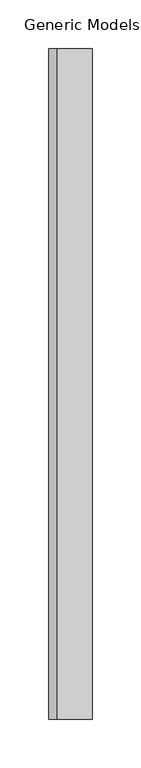
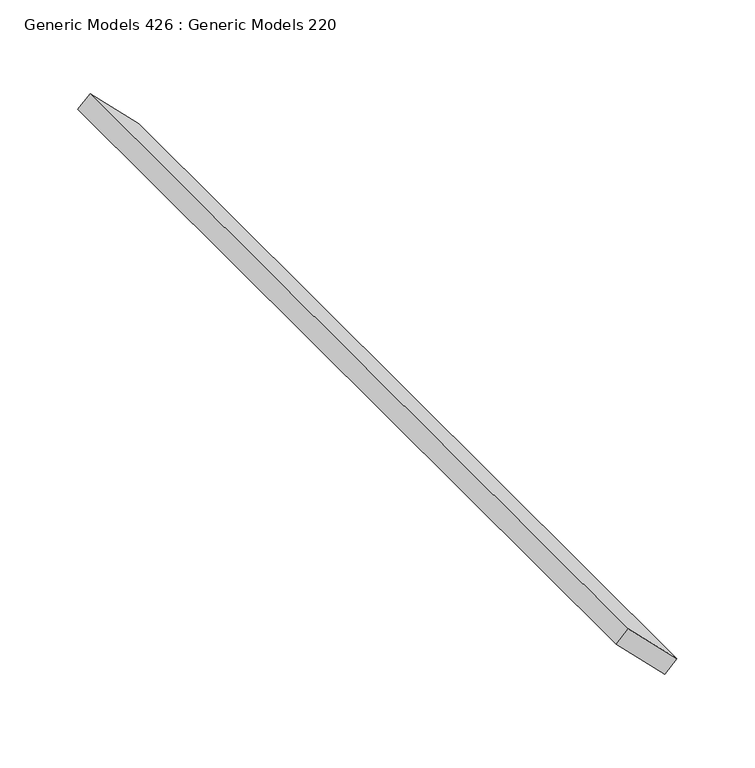
"""IFC4 building model written with IfcOpenShell, lengths in millimetres: proxy geometry, Generic Models 426 : Generic Models 220."""

from ifc_helpers import new_model, si_unit, frame, origin, place, context, project, spatial, polyline, outline, extrude, source, transform, mapped, element, save


def generic_models_426_generic_models_220_60b28b5c(model_context):
    return source(origin(), model_context, "Body", "SweptSolid", [
        extrude(outline(polyline([(0.0, -50.8), (0.0, 0.0), (690.8142348, 0.0), (690.8142348, -50.8), (0.0, -50.8)])), frame((-6899.085451, -4564.8872686, 128450.1762561), z_axis=(0.7071067811865582, 0.0, 0.7071067811865369), x_axis=(0.0, 1.0, 0.0)), (0.0, 0.0, 1.0), 12.7),
    ])


if __name__ == "__main__":
    model = new_model("IFC4")
    model_context = context("Model", 3, world=origin())
    ifc_project = project(units=[si_unit("LENGTHUNIT", "METRE", prefix="MILLI")], contexts=[model_context])
    site = spatial("IfcSite", under=ifc_project)
    building = spatial("IfcBuilding", under=site)
    placement = place(None, origin())
    generic_models_426_generic_models_220_shape = generic_models_426_generic_models_220_60b28b5c(model_context)
    element("IfcBuildingElementProxy", 1, Name="Generic Models 426 : Generic Models 220", ObjectType="Generic Models 426 : Generic Models 220", at=placement, inside=building, context=model_context, shape_type="MappedRepresentation", body=[
        mapped(generic_models_426_generic_models_220_shape, transform((0.0, 0.0, 0.0), x_axis=(1.0, 0.0, 0.0), y_axis=(0.0, 1.0, 0.0), z_axis=(0.0, 0.0, 1.0))),
    ])
    save(model, "model.ifc")

# Revit data of these elements
# Element 1 (IfcBuildingElementProxy, "Generic Models 426 : Generic Models 220")
#   Materials on its faces: "_WOOD TONE ALUMINUM EXTRUSION SLAT BY KNOTWOOD"
# Materials
#   "_WOOD TONE ALUMINUM EXTRUSION SLAT BY KNOTWOOD": class "Generic", colour RGB 177 130 114, transparency 0, Cost = 0
